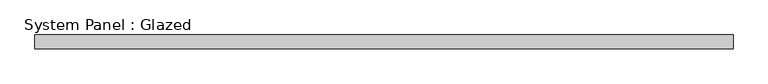
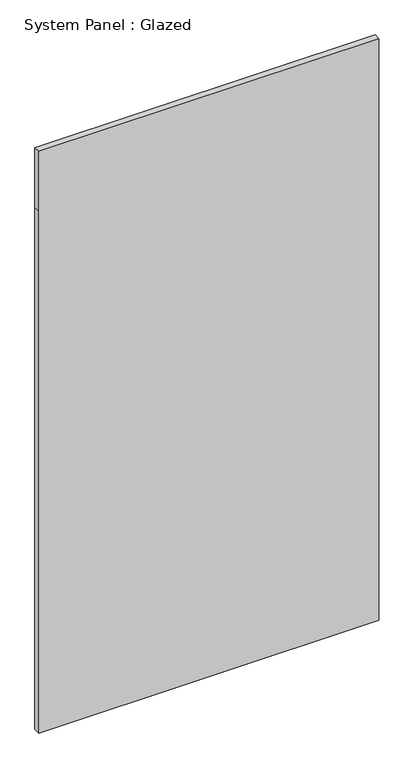
"""IFC4 building model written with IfcOpenShell, lengths in millimetres: plate geometry, System Panel : Glazed."""

import ifcopenshell
import ifcopenshell.guid

model = None  # the IFC model being written
_history = None  # IfcOwnerHistory: only IFC2X3 demands one
_inside = {}  # id of a spatial element -> (the spatial element, [elements in it])
_under = {}  # id of a project, library or spatial element -> (it, [spatial elements below it])
_declared = {}  # id of a project -> (the project, [libraries it declares])
_typed = {}  # id of a type object -> (the type object, [elements of that type])
_made_of = {}  # id of a material, layer set ... -> (it, [elements and type objects made of it])


def new_model(schema):
    """Start an empty IFC model of exactly this schema.

    Asked for "IFC4X3", IfcOpenShell would pick the latest addendum, in which some entities
    have other attributes; the version numbers below select the first issue.
    IFC2X3 requires an IfcOwnerHistory on every rooted entity: one is made here for all.
    """
    global model, _history
    if schema == "IFC4X3":
        model = ifcopenshell.file(schema_version=(4, 3, 0, 0))
    else:
        model = ifcopenshell.file(schema=schema)
    _inside.clear()
    _under.clear()
    _declared.clear()
    _typed.clear()
    _made_of.clear()
    _history = None
    if model.schema == "IFC2X3":
        org = make("IfcOrganization", Name="unknown")
        user = make(
            "IfcPersonAndOrganization",
            ThePerson=make("IfcPerson", FamilyName="unknown"),
            TheOrganization=org,
        )
        app = make(
            "IfcApplication",
            ApplicationDeveloper=org,
            Version="unknown",
            ApplicationFullName="unknown",
            ApplicationIdentifier="unknown",
        )
        _history = make(
            "IfcOwnerHistory",
            OwningUser=user,
            OwningApplication=app,
            ChangeAction="ADDED",
            CreationDate=0,
        )
    return model


def make(cls, **values):
    """One entity of the class cls with the attributes given. An attribute that is None is left unset."""
    return model.create_entity(
        cls, **{name: value for name, value in values.items() if value is not None}
    )


def rooted(cls, **values):
    """An entity with a GlobalId (a new one), such as an element, a storey or a relation."""
    return make(cls, GlobalId=ifcopenshell.guid.new(), OwnerHistory=_history, **values)


def si_unit(unit_type, name, prefix=None):
    """IfcSIUnit, for example si_unit("LENGTHUNIT", "METRE", prefix="MILLI")."""
    return make("IfcSIUnit", UnitType=unit_type, Prefix=prefix, Name=name)


def assignment(units):
    """IfcUnitAssignment: the units of a project."""
    return None if units is None else make("IfcUnitAssignment", Units=units)


def point(xyz):
    """IfcCartesianPoint."""
    return None if xyz is None else make("IfcCartesianPoint", Coordinates=xyz)


def direction(xyz):
    """IfcDirection."""
    return None if xyz is None else make("IfcDirection", DirectionRatios=xyz)


def frame(location, z_axis=None, x_axis=None):
    """IfcAxis2Placement3D, a coordinate frame: its origin and axes. An axis left out is left unset."""
    return make(
        "IfcAxis2Placement3D",
        Location=point(location),
        Axis=direction(z_axis),
        RefDirection=direction(x_axis),
    )


def origin():
    """The frame at (0, 0, 0) with its axes left unset."""
    return frame((0.0, 0.0, 0.0))


def place(relative_to, where):
    """IfcLocalPlacement: puts the frame where relative to a parent placement (None: the world)."""
    return make(
        "IfcLocalPlacement", PlacementRelTo=relative_to, RelativePlacement=where
    )


def context(
    kind, dimensions, precision=None, world=None, true_north=None, identifier=None
):
    """IfcGeometricRepresentationContext, for example the 3D "Model" context."""
    return make(
        "IfcGeometricRepresentationContext",
        ContextIdentifier=identifier,
        ContextType=kind,
        CoordinateSpaceDimension=dimensions,
        Precision=precision,
        WorldCoordinateSystem=world,
        TrueNorth=true_north,
    )


def project(units=None, contexts=None):
    """IfcProject with its units and contexts."""
    return rooted(
        "IfcProject",
        Name="project",
        RepresentationContexts=contexts,
        UnitsInContext=assignment(units),
    )


def spatial(cls, under=None, at=None, **own):
    """A site, building, storey or space (cls), placed at a placement, below another one or the project."""
    s = rooted(cls, ObjectPlacement=at, **own)
    if under is not None:
        _under.setdefault(under.id(), (under, []))[1].append(s)
    return s


def polyline(points):
    """IfcPolyline through the points."""
    return make("IfcPolyline", Points=[point(p) for p in points])


def outline(outer, holes=None, kind="AREA"):
    """IfcArbitraryClosedProfileDef: a profile drawn as a closed curve; with holes, ...WithVoids."""
    if holes is None:
        return make("IfcArbitraryClosedProfileDef", ProfileType=kind, OuterCurve=outer)
    return make(
        "IfcArbitraryProfileDefWithVoids",
        ProfileType=kind,
        OuterCurve=outer,
        InnerCurves=holes,
    )


def extrude(swept, where, along, depth):
    """IfcExtrudedAreaSolid: the profile swept, set in the frame where, extruded along a direction by depth."""
    return make(
        "IfcExtrudedAreaSolid",
        SweptArea=swept,
        Position=where,
        ExtrudedDirection=direction(along),
        Depth=depth,
    )


def shape(context_of_items, identifier, shape_type, items):
    """IfcShapeRepresentation: the items that make up one representation, for example the "Body"."""
    return make(
        "IfcShapeRepresentation",
        ContextOfItems=context_of_items,
        RepresentationIdentifier=identifier,
        RepresentationType=shape_type,
        Items=items,
    )


def source(mapping_origin, context_of_items, identifier, shape_type, items):
    """IfcRepresentationMap: a shape defined once, which mapped items show again and again."""
    return make(
        "IfcRepresentationMap",
        MappingOrigin=mapping_origin,
        MappedRepresentation=shape(context_of_items, identifier, shape_type, items),
    )


def transform(
    local_origin,
    x_axis=None,
    y_axis=None,
    z_axis=None,
    scale=None,
    scale2=None,
    scale3=None,
    uniform=True,
):
    """IfcCartesianTransformationOperator3D, or its non-uniform kind. x_axis, y_axis, z_axis: its Axis1, 2, 3."""
    if uniform:
        return make(
            "IfcCartesianTransformationOperator3D",
            Axis1=direction(x_axis),
            Axis2=direction(y_axis),
            LocalOrigin=point(local_origin),
            Scale=scale,
            Axis3=direction(z_axis),
        )
    return make(
        "IfcCartesianTransformationOperator3DnonUniform",
        Axis1=direction(x_axis),
        Axis2=direction(y_axis),
        LocalOrigin=point(local_origin),
        Scale=scale,
        Axis3=direction(z_axis),
        Scale2=scale2,
        Scale3=scale3,
    )


def mapped(mapping_source, mapping_target):
    """IfcMappedItem: shows the shape of a source again, moved by a transform."""
    return make(
        "IfcMappedItem", MappingSource=mapping_source, MappingTarget=mapping_target
    )


def made_of(thing, what):
    """Note that an element or type object is made of a material, layer set ...; save() writes the relation."""
    if what is not None:
        _made_of.setdefault(what.id(), (what, []))[1].append(thing)
    return thing


def element(
    cls,
    number,
    at=None,
    inside=None,
    cuts=None,
    type_object=None,
    material=None,
    context=None,
    identifier="Body",
    shape_type=None,
    held_by="IfcProductDefinitionShape",
    body=None,
    shapes=None,
    **own,
):
    """One element of the class cls, such as IfcWall. Its Tag is "e" and its number.

    at: its placement. inside: the storey or other place that contains it. cuts: it is an
    opening in that element (IfcRelVoidsElement). A single representation is given by context,
    identifier, shape_type and body (its items); several are given by shapes. held_by: the class
    of the entity that holds the representations. save() writes the other relations.
    """
    e = rooted(cls, Tag="e%d" % number, ObjectPlacement=at, **own)
    if body is not None:
        shapes = [shape(context, identifier, shape_type, body)]
    if shapes is not None:
        e.Representation = make(held_by, Representations=shapes)
    if inside is not None:
        _inside.setdefault(inside.id(), (inside, []))[1].append(e)
    if cuts is not None:
        rooted(
            "IfcRelVoidsElement", RelatingBuildingElement=cuts, RelatedOpeningElement=e
        )
    if type_object is not None:
        _typed.setdefault(type_object.id(), (type_object, []))[1].append(e)
    return made_of(e, material)


def aggregate(whole, parts):
    """IfcRelAggregates: a whole, such as a stair, and the parts it consists of."""
    return rooted("IfcRelAggregates", RelatingObject=whole, RelatedObjects=parts)


def save(model, path):
    """Write the relations noted so far, then the file.

    IfcRelAggregates (storeys below a building ...), IfcRelContainedInSpatialStructure (elements
    in a storey), IfcRelDefinesByType, IfcRelAssociatesMaterial and IfcRelDeclares: one each for
    every whole, place, type object, material and project.
    """
    for whole, parts in _under.values():
        aggregate(whole, parts)
    for where, things in _inside.values():
        rooted(
            "IfcRelContainedInSpatialStructure",
            RelatedElements=things,
            RelatingStructure=where,
        )
    for kind, things in _typed.values():
        rooted("IfcRelDefinesByType", RelatedObjects=things, RelatingType=kind)
    for what, things in _made_of.values():
        rooted("IfcRelAssociatesMaterial", RelatedObjects=things, RelatingMaterial=what)
    for by, libraries in _declared.values():
        rooted("IfcRelDeclares", RelatingContext=by, RelatedDefinitions=libraries)
    model.write(path)


def system_panel_glazed_c092dd15(model_context):
    return source(origin(), model_context, "Body", "SweptSolid", [
        extrude(outline(polyline([(0.0, -648.1535714), (0.0, 648.1535714), (2101.85, 648.1535714), (2343.15, 648.1535714), (2343.15, -648.1535714), (2101.85, -648.1535714), (0.0, -648.1535714)])), frame((0.0, 19.05, 0.0), z_axis=(0.0, 1.0, 0.0), x_axis=(0.0, 0.0, 1.0)), (0.0, 0.0, 1.0), 25.4),
    ])


if __name__ == "__main__":
    model = new_model("IFC4")
    model_context = context("Model", 3, world=origin())
    ifc_project = project(units=[si_unit("LENGTHUNIT", "METRE", prefix="MILLI")], contexts=[model_context])
    site = spatial("IfcSite", under=ifc_project)
    building = spatial("IfcBuilding", under=site)
    placement = place(None, origin())
    system_panel_glazed_shape = system_panel_glazed_c092dd15(model_context)
    element("IfcPlate", 1, ObjectType="System Panel : Glazed", at=placement, inside=building, context=model_context, shape_type="MappedRepresentation", body=[
        mapped(system_panel_glazed_shape, transform((0.0, 0.0, 0.0), x_axis=(1.0, 0.0, 0.0), y_axis=(0.0, 1.0, 0.0), z_axis=(0.0, 0.0, 1.0))),
    ])
    save(model, "model.ifc")

# Revit data of these elements
# Element 1 (IfcPlate, "System Panel : Glazed")
#   Materials on its faces: "Glass"
# Materials
#   "Glass": class "Glass", colour RGB 0 128 192, transparency 0.75
